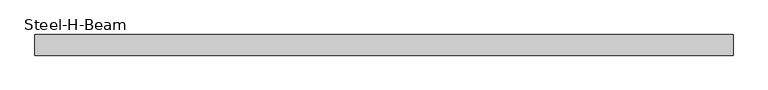
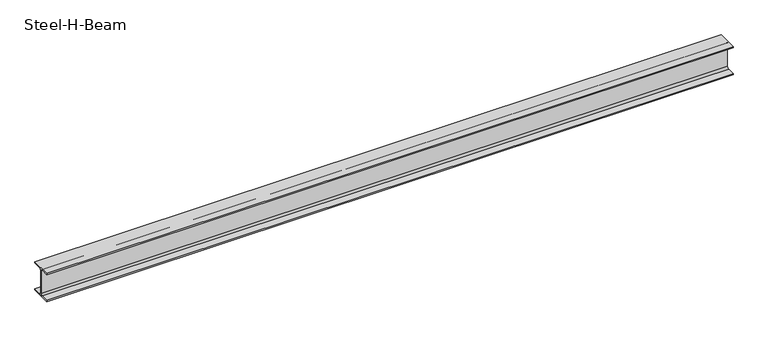
# IFC4 building model written with IfcOpenShell, lengths in millimetres: beam geometry, Steel-H-Beam : BM121_H-294×200x8x12.
# Revit data of these elements (continued)
# Project information (continued)
#     -cfd758078946\" /><element revit_id=\"af7cfdda-f71a-4a09-bb03-63e0c16d5d93-001530cf\" ism_id=\"46a5ded9-4fed-43a0-a06e-bb0fce603002\" /><element revit_id=\"af7cfdda-f71a-4a09-bb03-63e0c16d5d93-001530d1\" ism_id=\"62d05a0c-55f2-4c29-a355-b77f91c84c50\" /><element revit_id=\"af7cfdda-f71a-4a09-bb03-63e0c16d5d93-001530d3\" ism_id=\"eac0c420-7041-45a3-ad98-0cab4f5d8155\" /><element revit_id=\"af7cfdda-f71a-4a09-bb03-63e0c16d5d93-001530d5\" ism_id=\"9f5beb51-429a-4c7b-aa2e-ad2efe601ed6\" /><element revit_id=\"af7cfdda-f71a-4a09-bb03-63e0c16d5d93-001530d7\" ism_id=\"4613af3e-a189-4781-a937-106d789655c9\" /><element revit_id=\"af7cfdda-f71a-4a09-bb03-63e0c16d5d93-001530d9\" ism_id=\"71402e21-51c1-43b7-b8cc-75d2aba247eb\" /><element revit_id=\"af7cfdda-f71a-4a09-bb03-63e0c16d5d93-001530db\" ism_id=\"89101b83-9b84-4f11-b026-90cd564a3900\" /><element revit_id=\"af7cfdda-f71a-4a09-bb03-63e0c16d5d93-001530dd\" ism_id=\"37670781-ce23-4ce1-992b-7a400613c37b\" /><element revit_id=\"af7cfdda-f71a-4a09-bb03-63e0c16d5d93-001530df\" ism_id=\"2316856d-18eb-466b-8ab8-114816378db0\" /><element revit_id=\"af7cfdda-f71a-4a09-bb03-63e0c16d5d93-001530e2\" ism_id=\"da4f1597-5b5a-43a6-aa94-e478ffd6cfc7\" /><element revit_id=\"af7cfdda-f71a-4a09-bb03-63e0c16d5d93-001530e5\" ism_id=\"60805764-efb2-4434-8d81-aed3c3ed3c1b\" /><element revit_id=\"af7cfdda-f71a-4a09-bb03-63e0c16d5d93-001530e8\" ism_id=\"34e34ebb-6481-4bfb-b3d0-cb52295ff652\" /><element revit_id=\"af7cfdda-f71a-4a09-bb03-63e0c16d5d93-001530eb\" ism_id=\"dd5c4d73-1406-4c40-a955-5f9c52d01161\" /><element revit_id=\"af7cfdda-f71a-4a09-bb03-63e0c16d5d93-001530ed\" ism_id=\"cf8abc6b-638f-4bd5-8b66-615be032e220\" /><element revit_id=\"af7cfdda-f71a-4a09-bb03-63e0c16d5d93-001530f0\" ism_id=\"56ce8857-0c24-48d5-82f2-459e263998e2\" /><element revit_id=\"af7cfdda-f71a-4a09-bb03-63e0c16d5d93-001530f2\" ism_id=\"a1f000e8-ea08-442b-8a96-da7657653fd5\" /><element revit_id=\"af7cfdda-f71a-4a09-bb03-63e0c16d5d93-001530f4\" ism_id=\"2625e954-f7fb-41eb-b9bd-1b615ef945fc\" /><element revit_id=\"af7cfdda-f71a-4a09-bb03-63e0c16d5d93-001530f6\" ism_id=\"48469362-393c-4deb-bbb2-ad00180a23fb\" /><element revit_id=\"af7cfdda-f71a-4a09-bb03-63e0c16d5d93-001530f8\" ism_id=\"8e650f6f-0906-45a9-8fb8-35680155d6db\" /><element revit_id=\"af7cfdda-f71a-4a09-bb03-63e0c16d5d93-001530fb\" ism_id=\"f84acaf6-20a1-4df6-afed-1dc07fd0b2e9\" /><element revit_id=\"af7cfdda-f71a-4a09-bb03-63e0c16d5d93-001530fe\" ism_id=\"72816c7e-9128-47f4-b46a-ee567a2a03d6\" /><element revit_id=\"af7cfdda-f71a-4a09-bb03-63e0c16d5d93-00153100\" ism_id=\"c95ab0f8-b4bf-4b7c-bd1d-0423c8ac725a\" /><element revit_id=\"af7cfdda-f71a-4a09-bb03-63e0c16d5d93-00153102\" ism_id=\"32fd4119-6673-4973-aef2-b39ef90310e5\" /><element revit_id=\"af7cfdda-f71a-4a09-bb03-63e0c16d5d93-00153104\" ism_id=\"fd2aa4a6-d123-4100-85b9-db27c20cf6bc\" /><element revit_id=\"af7cfdda-f71a-4a09-bb03-63e0c16d5d93-00153106\" ism_id=\"e00fdefa-e77c-4406-9dbe-3c9122259821\" /><element revit_id=\"af7cfdda-f71a-4a09-bb03-63e0c16d5d93-00153108\" ism_id=\"25e5b79e-07c2-4ffa-a7a9-bf039dd2ad78\" /><element revit_id=\"af7cfdda-f71a-4a09-bb03-63e0c16d5d93-0015310b\" ism_id=\"720021d4-ca74-47c0-9c64-7d0854fa39f5\" /><element revit_id=\"af7cfdda-f71a-4a09-bb03-63e0c16d5d93-0015310d\" ism_id=\"ea922120-0cff-4f8d-a5c2-2841c031873e\" /><element revit_id=\"af7cfdda-f71a-4a09-bb03-63e0c16d5d93-0015310f\" ism_id=\"9d07ca73-3a65-44fe-ab61-476d8d1352d1\" /><element revit_id=\"af7cfdda-f71a-4a09-bb03-63e0c16d5d93-00153111\" ism_id=\"68a2fb30-d213-40c7-a166-dad5a20bd269\" /><element revit_id=\"af7cfdda-f71a-4a09-bb03-63e0c16d5d93-00153113\" ism_id=\"06119775-28f9-44f0-a265-5c57029016d1\" /><element revit_id=\"af7cfdda-f71a-4a09-bb03-63e0c16d5d93-00153115\" ism_id=\"ca133383-8253-4d07-aa92-f507fbb2ee47\" /><element revit_id=\"af7cfdda-f71a-4a09-bb03-63e0c16d5d93-00153117\" ism_id=\"6f4a7c07-4bd3-4c99-b1e4-110c964ccc07\" /><element revit_id=\"af7cfdda-f71a-4a09-bb03-63e0c16d5d93-00153119\" ism_id=\"ee1f865b-98a9-4ff1-a84c-52926e8f3566\" /><element revit_id=\"af7cfdda-f71a-4a09-bb03-63e0c16d5d93-0015311b\" ism_id=\"4fd7bd5c-7c46-4e79-a72b-dab4a1d98f33\" /><element revit_id=\"af7cfdda-f71a-4a09-bb03-63e0c16d5d93-0015311e\" ism_id=\"9ca0cac6-aaff-412a-b9c1-a8be985bc44a\" /><element revit_id=\"af7cfdda-f71a-4a09-bb03-63e0c16d5d93-00153121\" ism_id=\"73123639-76b5-46f0-a49e-b26af36d93b1\" /><element revit_id=\"af7cfdda-f71a-4a09-bb03-63e0c16d5d93-00153123\" ism_id=\"f74e8cb9-a93d-4aaa-985b-c0ed9befad19\" /><element revit_id=\"af7cfdda-f71a-4a09-bb03-63e0c16d5d93-00153126\" ism_id=\"5778daa1-b4cb-4cc3-9b7d-323562a47fba\" /><element revit_id=\"af7cfdda-f71a-4a09-bb03-63e0c16d5d93-00153129\" ism_id=\"2d7457d2-8978-4c95-9056-ebbaed3263eb\" /><element revit_id=\"af7cfdda-f71a-4a09-bb03-63e0c16d5d93-0015312c\" ism_id=\"48b420ce-6767-430a-aadc-695c25361a2d\" /><element revit_id=\"af7cfdda-f71a-4a09-bb03-63e0c16d5d93-0015312e\" ism_id=\"fc34038c-136d-4d55-b951-9cc35899fd33\" /><element revit_id=\"af7cfdda-f71a-4a09-bb03-63e0c16d5d93-00153130\" ism_id=\"e7a25938-3b91-4519-a48d-86fdd79489d5\" /><element revit_id=\"af7cfdda-f71a-4a09-bb03-63e0c16d5d93-00153133\" ism_id=\"c81dfd8c-579c-4d77-ab89-bf1f415d9cc6\" /><element revit_id=\"af7cfdda-f71a-4a09-bb03-63e0c16d5d93-00153136\" ism_id=\"5756a4b4-84ca-418c-b9f6-2d2370afca2f\" /><element revit_id=\"af7cfdda-f71a-4a09-bb03-63e0c16d5d93-0015313a\" ism_id=\"09a9cede-a757-4d8e-a722-6140af98bc61\" /><element revit_id=\"af7cfdda-f71a-4a09-bb03-63e0c16d5d93-0015313d\" ism_id=\"ac9b583c-7f63-4351-8b69-3967279b234c\" /><element revit_id=\"af7cfdda-f71a-4a09-bb03-63e0c16d5d93-00153140\" ism_id=\"1a52584d-6b21-4de6-bb42-5b9bdd6f24e9\" /><element revit_id=\"af7cfdda-f71a-4a09-bb03-63e0c16d5d93-00153143\" ism_id=\"6c2e2bc0-8432-4c98-9292-cbb2182bd4b0\" /><element revit_id=\"af7cfdda-f71a-4a09-bb03-63e0c16d5d93-00153145\" ism_id=\"644bb900-7654-42c5-a9b7-996a2197f6d0\" /><element revit_id=\"af7cfdda-f71a-4a09-bb03-63e0c16d5d93-00153148\" ism_id=\"a1bca0bd-75db-464c-b27a-2a69d9b4ad3d\" /><element revit_id=\"af7cfdda-f71a-4a09-bb03-63e0c16d5d93-0015314a\" ism_id=\"ea29955b-34f2-409a-aefa-e6adfe75349e\" /><element revit_id=\"af7cfdda-f71a-4a09-bb03-63e0c16d5d93-0015314d\" ism_id=\"800fef33-e5e1-422c-b708-e9394bbeefcc\" /><element revit_id=\"af7cfdda-f71a-4a09-bb03-63e0c16d5d93-0015314f\" ism_id=\"86259dca-8773-4253-ac56-e71252267c8a\" /><element revit_id=\"af7cfdda-f71a-4a09-bb03-63e0c16d5d93-00153152\" ism_id=\"d15a0ad2-db9f-420d-bea3-41a78a0eb330\" /><element revit_id=\"af7cfdda-f71a-4a09-bb03-63e0c16d5d93-00153155\" ism_id=\"bd27f420-df49-4abe-bd96-8e48e7f4efcb\" /><element revit_id=\"af7cfdda-f71a-4a09-bb03-63e0c16d5d93-00153157\" ism_id=\"5d451f94-860d-4cc3-a4fa-51a9f3126e33\" /><element revit_id=\"af7cfdda-f71a-4a09-bb03-63e0c16d5d93-0015315a\" ism_id=\"4234158a-994a-492b-85da-6108709b7232\" /><element revit_id=\"af7cfdda-f71a-4a09-bb03-63e0c16d5d93-0015315c\" ism_id=\"ca24c92d-986b-417f-812f-024ab15e24c8\" /><element revit_id=\"af7cfdda-f71a-4a09-bb03-63e0c16d5d93-0015315f\" ism_id=\"699ec3b0-0151-4110-b054-14418651f324\" /><element revit_id=\"af7cfdda-f71a-4a09-bb03-63e0c16d5d93-00153161\" ism_id=\"38ecdeac-3d85-48dd-82c1-53fe93f49beb\" /><element revit_id=\"af7cfdda-f71a-4a09-bb03-63e0c16d5d93-00153163\" ism_id=\"1340aefd-b79c-4264-8a49-d0a0504eff8c\" /><element revit_id=\"af7cfdda-f71a-4a09-bb03-63e0c16d5d93-00153165\" ism_id=\"1b6167c2-fb26-4b8d-916b-d835d89896e7\" /><element revit_id=\"af7cfdda-f71a-4a09-bb03-63e0c16d5d93-00153167\" ism_id=\"290d3d83-57eb-4125-aecb-a977a5fcf5ca\" /><element revit_id=\"af7cfdda-f71a-4a09-bb03-63e0c16d5d93-00153169\" ism_id=\"105c9b97-1c70-4237-82ac-8404a3e8e6a6\" /><element revit_id=\"af7cfdda-f71a-4a09-bb03-63e0c16d5d93-0015316c\" ism_id=\"1726c5bb-05e2-4959-9da2-4227f0219f00\" /><element revit_id=\"af7cfdda-f71a-4a09-bb03-63e0c16d5d93-0015316e\" ism_id=\"d919ee9c-caed-4119-b451-e3644db952c8\" /><element revit_id=\"af7cfdda-f71a-4a09-bb03-63e0c16d5d93-00153170\" ism_id=\"1b1fab26-60c4-40ed-b31b-b177eda246ce\" /><element revit_id=\"af7cfdda-f71a-4a09-bb03-63e0c16d5d93-00153172\" ism_id=\"ea9b5221-a1f2-4796-8cca-f7872ab69cbd\" /><element revit_id=\"af7cfdda-f71a-4a09-bb03-63e0c16d5d93-00153174\" ism_id=\"660b40b2-06fb-4b62-b987-28a171e473fe\" /><element revit_id=\"af7cfdda-f71a-4a09-bb03-63e0c16d5d93-00153176\" ism_id=\"767be0d9-c5ba-4ad3-a52d-efd60031fc9a\" /><element revit_id=\"af7cfdda-f71a-4a09-bb03-63e0c16d5d93-00153178\" ism_id=\"6fbe93ce-4ed7-4596-88fc-71dafe48803e\" /><element revit_id=\"af7cfdda-f71a-4a09-bb03-63e0c16d5d93-0015317a\" ism_id=\"27d7b093-4eb7-47aa-b123-5388a6327d7f\" /><element revit_id=\"af7cfdda-f71a-4a09-bb03-63e0c16d5d93-0015317c\" ism_id=\"9073a947-5952-42fe-b37a-cdfed3ca30c7\" /><element revit_id=\"af7cfdda-f71a-4a09-bb03-63e0c16d5d93-0015317e\" ism_id=\"1888f060-aa3c-4494-8f30-a80ca2311216\" /><element revit_id=\"af7cfdda-f71a-4a09-bb03-63e0c16d5d93-00153181\" ism_id=\"c0491dc2-5df2-4c14-b988-e117f6f511a2\" /><element revit_id=\"af7cfdda-f71a-4a09-bb03-63e0c16d5d93-00153184\" ism_id=\"4f44b9aa-c092-46fe-bf9b-2d1be872d419\" /><element revit_id=\"af7cfdda-f71a-4a09-bb03-63e0c16d5d93-00153186\" ism_id=\"eb560801-76cf-40a8-a181-31cd32aca14f\" /><element revit_id=\"af7cfdda-f71a-4a09-bb03-63e0c16d5d93-00153189\" ism_id=\"8d1e5f00-41d5-42c1-9b4f-a8c2eb689a72\" /><element revit_id=\"af7cfdda-f71a-4a09-bb03-63e0c16d5d93-0015318b\" ism_id=\"caf6c2dc-0e9e-46a9-a3e1-71316081ff61\" /><element revit_id=\"af7cfdda-f71a-4a09-bb03-63e0c16d5d93-0015318d\" ism_id=\"4d149f88-f5b9-4943-8765-090324e0a65d\" /><element revit_id=\"af7cfdda-f71a-4a09-bb03-63e0c16d5d93-0015318f\" ism_id=\"75865cf2-3adc-4a52-a778-fc6fb65fcdcb\" /><element revit_id=\"af7cfdda-f71a-4a09-bb03-63e0c16d5d93-00153191\" ism_id=\"f9320017-2083-48f1-8aff-e6ba958fb1c5\" /><element revit_id=\"af7cfdda-f71a-4a09-bb03-63e0c16d5d93-00153193\" ism_id=\"38a61c12-98f2-47b1-843d-8351040e24d2\" /><element revit_id=\"af7cfdda-f71a-4a09-bb03-63e0c16d5d93-00153196\" ism_id=\"af709a9c-b664-480b-be0d-fb01aac630f2\" /><element revit_id=\"af7cfdda-f71a-4a09-bb03-63e0c16d5d93-00153199\" ism_id=\"a4c2867c-ca2a-4112-b86c-4e6563e3dc63\" /><element revit_id=\"14a48413-84c4-4e00-9e64-4f618415469a-0013ce74\" ism_id=\"F2ADF140-E21A-4820-8170-6F63D956DCAD\" /><element revit_id=\"14a48413-84c4-4e00-9e64-4f618415469a-0013ce74\" ism_id=\"B35A310E-4F33-462b-819C-3ADD300C0CEB\" /><element revit_id=\"14a48413-84c4-4e00-9e64-4f618415469a-0013ce74\" ism_id=\"711054EC-0DB2-46e3-AD20-004560300C00\" /><element revit_id=\"14a48413-84c4-4e00-9e64-4f618415469a-0013ce6e\" ism_id=\"B5C54EC9-8EBD-4860-AB72-EF5791AED394\" /><element revit_id=\"14a48413-84c4-4e00-9e64-4f618415469a-0013e793\" ism_id=\"0A7B8D02-9EA4-4aa9-A41A-E30BB5B6B6C5\" /><element revit_id=\"14a48413-84c4-4e00-9e64-4f618415469a-0013e793\" ism_id=\"714BBD27-DB58-47da-B54C-5806291C2D3C\" /><element revit_id=\"14a48413-84c4-4e00-9e64-4f618415469a-0013e793\" ism_id=\"F36E62C1-13EE-4807-A3C1-899E23E0BEDE\" /><element revit_id=\"14a48413-84c4-4e00-9e64-4f618415469a-0013e793\" ism_id=\"F5448801-679E-44d6-8F46-E676344F8165\" /><element revit_id=\"14a48413-84c4-4e00-9e64-4f618415469a-0013e793\" ism_id=\"846DCB0C-E06B-4978-9D43-E1CC0FDE7595\" /><element revit_id=\"14a48413-84c4-4e00-9e64-4f618415469a-0013e793\" ism_id=\"2ADF82B8-986D-4f44-85DE-89D921292160\" /><element revit_id=\"14a48413-84c4-4e00-9e64-4f618415469a-0013e793\" ism_id=\"7AF371ED-051B-4a30-8826-11F11C212B73\" /><element revit_id=\"14a48413-84c4-4e00-9e64-4f618415469a-0013e793\" ism_id=\"2FE74006-ADDA-412f-A522-853919E62B4D\" /><element revit_id=\"14a48413-84c4-4e00-9e64-4f618415469a-0013e793\" ism_id=\"09B63641-D581-4a6c-A18E-54C17EC989A4\" /><element revit_id=\"14a48413-84c4-4e00-9e64-4f618415469a-0013e793\" ism_id=\"0DD6B52A-77D0-45a1-82B1-8236ED57078C\" /><element revit_id=\"14a48413-84c4-4e00-9e64-4f618415469a-0013e793\" ism_id=\"35D311D2-DEB8-4469-97DE-110B6DF5B84D\" /><element revit_id=\"14a48413-84c4-4e00-9e64-4f618415469a-0013e79
#     3\" ism_id=\"0D3CCDE5-CFF9-431b-A4BD-01BF6636D6BD\" /><element revit_id=\"14a48413-84c4-4e00-9e64-4f618415469a-0013e793\" ism_id=\"C62B2A5B-024A-47ac-B030-C17A67E64A7B\" /><element revit_id=\"14a48413-84c4-4e00-9e64-4f618415469a-0013e793\" ism_id=\"944C6E43-E607-48c3-8358-9E6CB88346E7\" /><element revit_id=\"14a48413-84c4-4e00-9e64-4f618415469a-0013e793\" ism_id=\"A4B1F42D-B1C2-4ad2-8AD6-DB0D5E05998D\" /><element revit_id=\"14a48413-84c4-4e00-9e64-4f618415469a-0013e793\" ism_id=\"007E6C70-1139-4b48-B003-C76FAD4C249A\" /><element revit_id=\"14a48413-84c4-4e00-9e64-4f618415469a-0013e793\" ism_id=\"9941AC94-F03A-464c-9912-04590E0C31E0\" /><element revit_id=\"14a48413-84c4-4e00-9e64-4f618415469a-0013e793\" ism_id=\"CFD98B8D-8FF4-4e71-A909-0FE7DBCE924E\" /><element revit_id=\"14a48413-84c4-4e00-9e64-4f618415469a-0013e793\" ism_id=\"58262161-98E6-45c8-B2BD-4508105FF662\" /><element revit_id=\"14a48413-84c4-4e00-9e64-4f618415469a-0013e793\" ism_id=\"66AB4841-610A-4883-97F7-1282A56484E1\" /><element revit_id=\"14a48413-84c4-4e00-9e64-4f618415469a-0013e793\" ism_id=\"D2B324BE-BBD6-49da-9730-60EA7AD4D3A0\" /><element revit_id=\"14a48413-84c4-4e00-9e64-4f618415469a-0013e793\" ism_id=\"92A8ECE7-C053-46b1-92ED-F2C041617E7B\" /><element revit_id=\"14a48413-84c4-4e00-9e64-4f618415469a-0013e793\" ism_id=\"B4C4BDB0-65C4-4016-9C78-DBD77E229523\" /><element revit_id=\"14a48413-84c4-4e00-9e64-4f618415469a-0013e793\" ism_id=\"57270646-162F-4c83-BDB7-A5FBEA9120BD\" /><element revit_id=\"14a48413-84c4-4e00-9e64-4f618415469a-0013e793\" ism_id=\"BDEF733F-00AA-4eee-B6C6-50229FC1D236\" /><element revit_id=\"14a48413-84c4-4e00-9e64-4f618415469a-0013e793\" ism_id=\"84A94E1E-3074-40f4-9690-97191755F019\" /><element revit_id=\"14a48413-84c4-4e00-9e64-4f618415469a-0013e793\" ism_id=\"8A7D913D-7967-4718-912D-B83DF0AD2EDD\" /><element revit_id=\"14a48413-84c4-4e00-9e64-4f618415469a-0013e793\" ism_id=\"83553D70-90FA-469c-B5C3-EF03F3FC6475\" /><element revit_id=\"14a48413-84c4-4e00-9e64-4f618415469a-0013e793\" ism_id=\"6880C1E4-C50B-4c1b-B61C-23F2D8C46873\" /><element revit_id=\"14a48413-84c4-4e00-9e64-4f618415469a-0013e793\" ism_id=\"08594C43-CD40-47de-A3BA-8BFB47F64994\" /><element revit_id=\"14a48413-84c4-4e00-9e64-4f618415469a-0013e793\" ism_id=\"7D2E11FA-A5E1-4434-B9BE-AABA1A16CA03\" /><element revit_id=\"14a48413-84c4-4e00-9e64-4f618415469a-0013e793\" ism_id=\"D892DFA4-5441-4ad2-A390-253492293B1B\" /><element revit_id=\"14a48413-84c4-4e00-9e64-4f618415469a-0013e793\" ism_id=\"E5A32FE6-89C4-49f1-B3B9-1CABE7C48A4D\" /><element revit_id=\"14a48413-84c4-4e00-9e64-4f618415469a-0013e793\" ism_id=\"8AE872C2-5DBE-47c5-934B-7E964A84B589\" /><element revit_id=\"14a48413-84c4-4e00-9e64-4f618415469a-0013e793\" ism_id=\"3C847B60-488A-4604-A400-16A3A65E919B\" /><element revit_id=\"14a48413-84c4-4e00-9e64-4f618415469a-0013e793\" ism_id=\"DBEC432A-3F7B-4266-AD99-2A937DC70BCF\" /><element revit_id=\"14a48413-84c4-4e00-9e64-4f618415469a-0013e793\" ism_id=\"59403DD6-7A51-48aa-A3BE-962457E6F10E\" /><element revit_id=\"14a48413-84c4-4e00-9e64-4f618415469a-0013e793\" ism_id=\"11CDDF5D-38B6-43b2-A291-FC188BE232BC\" /><element revit_id=\"14a48413-84c4-4e00-9e64-4f618415469a-0013e793\" ism_id=\"10BF2843-EFC9-4136-933C-5B270D970277\" /><element revit_id=\"14a48413-84c4-4e00-9e64-4f618415469a-0013e793\" ism_id=\"E1B09A9C-F6C6-47d9-976B-E313C0E3F52B\" /><element revit_id=\"14a48413-84c4-4e00-9e64-4f618415469a-0013e793\" ism_id=\"A3A22EC3-26C8-4588-A0AB-AFAE02DF267E\" /><element revit_id=\"14a48413-84c4-4e00-9e64-4f618415469a-0013e793\" ism_id=\"114828FC-BDC1-4343-9119-BCB5395DAA64\" /><element revit_id=\"14a48413-84c4-4e00-9e64-4f618415469a-0013e793\" ism_id=\"797626F9-3558-4623-826F-15FB93088CB3\" /><element revit_id=\"14a48413-84c4-4e00-9e64-4f618415469a-0013e793\" ism_id=\"4BF369CD-DF09-4346-96CB-C6C6380A2599\" /><element revit_id=\"14a48413-84c4-4e00-9e64-4f618415469a-0013e793\" ism_id=\"722B46BA-61C4-44a1-9ECF-325B60B6688D\" /><element revit_id=\"14a48413-84c4-4e00-9e64-4f618415469a-0013e793\" ism_id=\"C33DBE84-19C1-4379-AB6E-A41F7420F18C\" /><element revit_id=\"14a48413-84c4-4e00-9e64-4f618415469a-0013e793\" ism_id=\"1F2D3B75-66F2-4d88-A1DD-647969477B86\" /><element revit_id=\"14a48413-84c4-4e00-9e64-4f618415469a-0013e793\" ism_id=\"DFBF96B2-410A-4f39-80C4-D8CF78561C93\" /><element revit_id=\"14a48413-84c4-4e00-9e64-4f618415469a-0013e793\" ism_id=\"D6793CD3-AB64-417c-9C28-8B18A0A2D336\" /><element revit_id=\"14a48413-84c4-4e00-9e64-4f618415469a-0013e793\" ism_id=\"90884AC0-EA00-4caa-86E1-E6B886FD90ED\" /><element revit_id=\"14a48413-84c4-4e00-9e64-4f618415469a-0013e793\" ism_id=\"64BC7B89-F7C8-4dae-A5C8-F10DF9E5F6BA\" /><element revit_id=\"14a48413-84c4-4e00-9e64-4f618415469a-0013e793\" ism_id=\"D82E4D85-2728-40e5-9F60-1C7FB2990D78\" /><element revit_id=\"14a48413-84c4-4e00-9e64-4f618415469a-0013e793\" ism_id=\"1E6D05B9-BF84-4669-AA27-948ADA1D511E\" /><element revit_id=\"14a48413-84c4-4e00-9e64-4f618415469a-0013e793\" ism_id=\"73608CB2-EB94-466e-883D-814030EF49D6\" /><element revit_id=\"14a48413-84c4-4e00-9e64-4f618415469a-0013e793\" ism_id=\"4EAF07EF-4E08-4065-9F08-BF69D4413867\" /><element revit_id=\"14a48413-84c4-4e00-9e64-4f618415469a-0013e0e9\" ism_id=\"05D74241-6318-4cac-95F5-7B878260D5B5\" /></element_binding><reinforcement_properties /><operation_settings><coordinate_mapping x=\"0\" y=\"0\" z=\"0\" /></operation_settings></ism>"
#   Building Name = "FIRE WATER PUMP BUILDING"
#   Project Status = "Project Status"
#   Client Name = "현대엔지니어링"
#   Project Address = "서울시 종로구 율곡로 75(계동)"
#   Project Name = "TAKHIATASH POWER PLANT EFFICIENCY IMPROVEMENT PROJECT / 우즈베키스탄"
#   Project Number = "BEUZ1602"
#   F01) Building Name = "FIRE WATER PUMP BUILDING"
#   F11) Project Building Tag_Type-1 = "BI aWBS"
#   F12) Project Building Tag_Type-2 = "BI aWBS"
#   F13) Project Facility Code = "621"
#   F21) Structural Type = "STEEL"
#   F31) Standard Building Code = "E204"
#   F41) Discipline = "Architecture"
#   F51) Plan Start Date-Engineering = "2018-01-01"
#   F52) Plan Finish Date-Engineering = "2018-09-13"
#   F53) Duration = "255"
#   F61) Plan Start Date-Construction = "2018-09-14"
#   F62) Plan Finish Date-Construction = "2019-12-02"
#   F63) Duration = "444"
#   F91) Plant Type = "2GTG+2STG+1HRSG"
#   F92) KKS Structures, Building = "UAB"
#   P01) Project Name = "TAKHIATASH POWER PLANT EFFICIENCY IMPROVEMENT PROJECT / 우즈베키스탄"
#   P02) Project Configuration = "2 GTG + 2 HRSG + 2STG, 2 x 250MW"
#   P03) Project Abbreviation = "UTCC"
#   P04) Project Code = "BEUZ1602"
#   P05) Project Stage = "실행"
#   P06) Project Location = "Takhiatash / Uzbekistan"
#   P07) Project Owner = "우즈베키스탄 전력청"
#   P08) Project O.E = "GAS Natural Fenosa"
#   P09) Project Schedule = "2017.10.01 ~ 2020.08.08"
#   P10) Basic Wind Speed = "48m/sec_ASCE7-05"
#   P11) Seismic = "SDS_0.15_ASCE7-05"
#   P12) Soil = "SD_ASCE7-05"
#   P13) Soil Capacity = "400 kN/m2_Soil Replacement"
#   P14) Pile Capacity = "1000 kN_D600 Board Pile"
# Type "Steel-H-Beam : BM121_H-294×200x8x12"
#   Surface Area = 1.3411 m²/m
#   Section Area = 72.3812 cm²
#   Mass per Unit Length = 56.8193 kg/m
#   Length [instance default] = 3000 mm
#   B = 200 mm
#   H = 294 mm
#   r = 18 mm
#   tw = 8 mm
#   tf = 12 mm
#   hec_material4 [instance default] = none
#   hec_material3 [instance default] = none
#   hec_material2 [instance default] = none
#   hec_material1 [instance default] = none
#   Structural Material [instance default] = Steel, 45-345
#   Assembly Code = ""
# Element 1 (IfcBeam, "Steel-H-Beam : BM121_H-294×200x8x12")
#   hec_material3 = F01AC000-00002_Building/Shelter Fire Proofing Work_Intumescent Coating Type_1 hr. rating (UL 1709))
#   hec_material2 = S01AA010-00002_Main Steel Structure Fabrication Work_Shelter/Building_Steel Painting/Coating_for Fireproofed Steel Surface, Surface Preparation & Primer Coat
#   hec_material1 = S03AA028-00001_Main Steel Structure Erection Work_Shelter/Building_Medium Steel
#   Structural Material = S01AA002-00001_Main Steel Structure Fabrication Work_Shelter/Building_Medium Steel - Standard
#   Materials on its faces: "S01AA002-00001_Main Steel Structure Fabrication Work_Shelter/Building_Medium Steel - Standard"
# Materials
#   "Steel, 45-345": class "Metal", colour RGB 189 187 185, transparency 0, Description = "Steel 345 MPa", Cost = 0
#   "S01AA002-00001_Main Steel Structure Fabrication Work_Shelter/Building_Medium Steel - Standard": class "Metal", colour RGB 120 120 120, transparency 0, Comments = "(90KG/M>Weight≥30KG/M)", Description = "Structural steel 50ksi", W00) Work Master Code = "S01AA002-0001", W01) Work Master_Lv1 = "Main Steel Structure Fabrication Work", W02) Work Master_Lv2 = "Shelter/Building", W03) Work Master_Spec.1 = "Medium Steel - Standard (90KG/M>Weight≥30KG/M)", Cost = 0
#   "F01AC000-00002_Building/Shelter Fire Proofing Work_Intumescent Coating Type_1 hr. rating (UL 1709))": class "Metal", colour RGB 255 128 128, transparency 0, Description = "Paint finished steel", W00) Work Master Code = "F01AC000-00002", W01) Work Master_Lv1 = "Building/Shelter Fire Proofing Work", W02) Work Master_Lv2 = "Intumescent Coating Type", W03) Work Master_Spec.1 = "1 hr. rating (UL 1709)", Cost = 0
#   "S01AA010-00002_Main Steel Structure Fabrication Work_Shelter/Building_Steel Painting/Coating_for Fireproofed Steel Surface, Surface Preparation & Primer Coat": class "Metal", colour RGB 120 120 120, transparency 0, Description = "Paint finished steel", W00) Work Master Code = "SS01AA010-00002", W01) Work Master_Lv1 = "Main Steel Structure Fabrication Work", W02) Work Master_Lv2 = "Shelter/Building", W03) Work Master_Spec.1 = "Steel Painting/Coating", W04) Work Master_Spec.2 = "for Fireproofed Steel Surface, Surface Preparation & Primer Coat", Cost = 0
#   "S03AA028-00001_Main Steel Structure Erection Work_Shelter/Building_Medium Steel": class "Metal", colour RGB 120 120 120, transparency 0, Comments = "(90KG/M>Weight≥30KG/M)", Description = "Structural steel 50ksi", W00) Work Master Code = "S03AA028-0001", W01) Work Master_Lv1 = "Main Steel Structure Erection Work", W02) Work Master_Lv2 = "Shelter/Building", W03) Work Master_Spec.1 = "Medium Steel (90KG/M>Weight≥30KG/M)", Cost = 0
